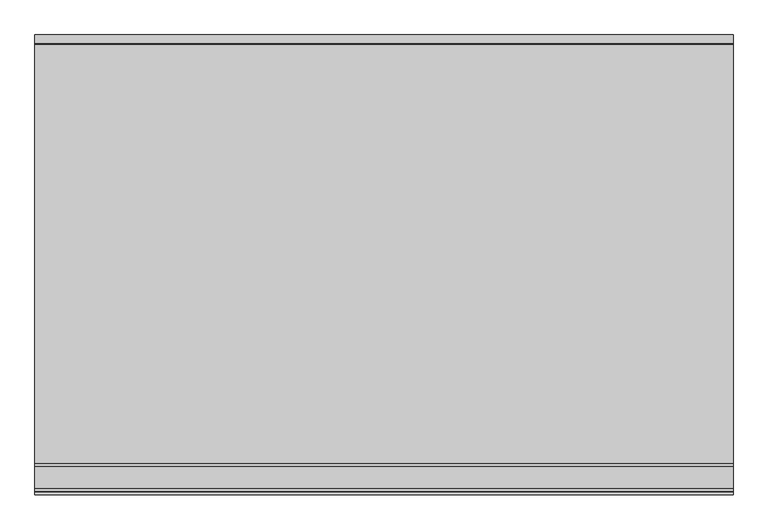
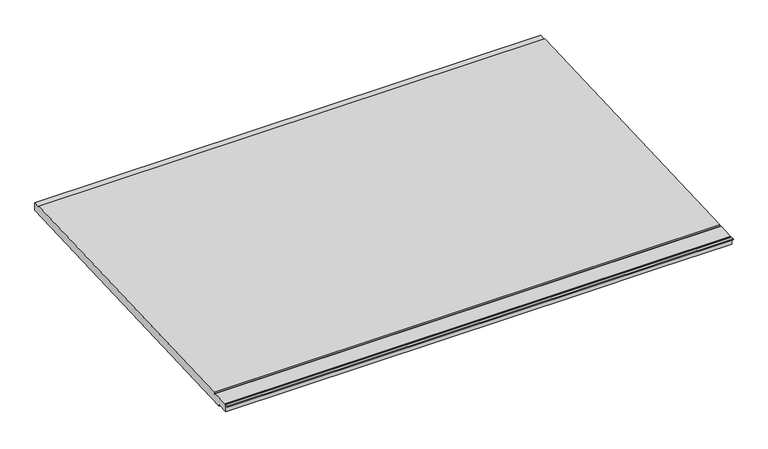
"""IFC4 building model written with IfcOpenShell, lengths in millimetres: proxy geometry, Generic Models 7:Generic Models 1:2:Generic Models 1:2 : Generic Models 7:Generic Models 1:337419:11 : Generic Models 7:Generic Models 1:2:Generic Models 1:2 : Generic Models 7:Generic Models 1:337419:306751."""

from ifc_helpers import new_model, si_unit, origin, place, context, project, spatial, faceted_brep, source, transform, mapped, element, save


def generic_models_fd5f59f4(model_context):
    return source(origin(), model_context, "Body", "Brep", [
        faceted_brep([(596182.8367239, -578988.1721757, 3950.4199851), (596182.8367239, -579061.0480378, 3947.3834909), (596182.8367239, -579059.461914, 3909.3165208), (596182.8367239, -578989.2957788, 3912.2401097), (596182.8367239, -578989.2957788, 3721.5748169), (596182.8367239, -578614.4804524, 3737.1921222), (596182.8367239, -578612.3656208, 3686.436162), (596182.8367239, -568205.6913841, 4120.0475886), (596182.8367239, -568205.6913841, 4374.267979), (596182.8367239, -568407.8188757, 4365.8460002), (596182.8367239, -568426.430308, 4390.492563), (596182.8367239, -578321.4396124, 3978.2005086), (596182.8367239, -578321.4396124, 3940.06745), (596182.8367239, -578397.8238233, 3936.8847746), (596182.8367239, -578397.8238233, 3975.0178331), (596182.8367239, -578911.9452054, 3953.5961089), (596182.8367239, -578910.3590816, 3915.5291388), (596182.8367239, -578986.5860519, 3912.353015), (579695.8219605, -579061.0480378, 3947.3834909), (579695.8219605, -578988.1721757, 3950.4199851), (579695.8219605, -578986.5860519, 3912.353015), (579695.8219605, -578910.3590816, 3915.5291388), (579695.8219605, -578911.9452054, 3953.5961089), (579695.8219605, -578397.8238233, 3975.0178331), (579695.8219605, -578397.8238233, 3936.8847746), (579695.8219605, -578321.4396124, 3940.06745), (579695.8219605, -578321.4396124, 3978.2005086), (579695.8219605, -568426.430308, 4390.492563), (579695.8219605, -568407.8188757, 4365.8460002), (579695.8219605, -568205.6913841, 4374.267979), (579695.8219605, -568205.6913841, 4120.0475886), (579695.8219605, -578612.3656208, 3686.436162), (579695.8219605, -578614.4804524, 3737.1921222), (579695.8219605, -578989.2957788, 3721.5748169), (579695.8219605, -578989.2957788, 3912.2401097), (579695.8219605, -579059.461914, 3909.3165208), (591306.0367239, -578989.2957788, 3721.5748169), (593738.0867239, -578989.2957788, 3721.5748169)], [[[0, 1, 2, 3, 4, 5, 6, 7, 8, 9, 10, 11, 12, 13, 14, 15, 16, 17]], [[18, 19, 20, 21, 22, 23, 24, 25, 26, 27, 28, 29, 30, 31, 32, 33, 34, 35]], [[1, 0, 19, 18]], [[9, 8, 29, 28]], [[10, 9, 28, 27]], [[8, 7, 30, 29]], [[7, 6, 31, 30]], [[2, 1, 18, 35]], [[3, 2, 35, 34]], [[4, 3, 34, 33, 36, 37]], [[5, 4, 37, 36, 33, 32]], [[6, 5, 32, 31]], [[15, 14, 23, 22]], [[16, 15, 22, 21]], [[17, 16, 21, 20]], [[0, 17, 20, 19]], [[11, 10, 27, 26]], [[12, 11, 26, 25]], [[13, 12, 25, 24]], [[14, 13, 24, 23]]]),
    ])


if __name__ == "__main__":
    model = new_model("IFC4")
    model_context = context("Model", 3, world=origin())
    ifc_project = project(units=[si_unit("LENGTHUNIT", "METRE", prefix="MILLI")], contexts=[model_context])
    site = spatial("IfcSite", under=ifc_project)
    building = spatial("IfcBuilding", under=site)
    placement = place(None, origin())
    generic_models_shape = generic_models_fd5f59f4(model_context)
    element("IfcBuildingElementProxy", 1, Name="Generic Models 7:Generic Models 1:2:Generic Models 1:2 : Generic Models 7:Generic Models 1:337419:11 : Generic Models 7:Generic Models 1:2:Generic Models 1:2 : Generic Models 7:Generic Models 1:337419:306751", ObjectType="Generic Models 7:Generic Models 1:2:Generic Models 1:2 : Generic Models 7:Generic Models 1:337419:11 : Generic Models 7:Generic Models 1:2:Generic Models 1:2 : Generic Models 7:Generic Models 1:337419:306751", at=placement, inside=building, context=model_context, shape_type="MappedRepresentation", body=[
        mapped(generic_models_shape, transform((0.0, 0.0, 0.0), x_axis=(1.0, 0.0, 0.0), y_axis=(0.0, 1.0, 0.0), z_axis=(0.0, 0.0, 1.0))),
    ])
    save(model, "model.ifc")

# Revit data of these elements
# Type "Generic Models 7:Generic Models 1:2:Generic Models 1:2 : Generic Models 7:Generic Models 1:337419:11 : Generic Models 7:Generic Models 1:2:Generic Models 1:2 : Generic Models 7:Generic Models 1:337419:306751"
#   NameOverride = "Generic Models 7:Generic Models 1:2:Generic Models 1:2 : Generic Models 7:Generic Models 1:337419:306751"
#   ObjectTypeOverride = "Generic Models 1:2 : Generic Models 7:Generic Models 1:337419"
#   Reference = "Generic Models 1"
#   Tag = "306751"
# Element 1 (IfcBuildingElementProxy, "Generic Models 7:Generic Models 1:2:Generic Models 1:2 : Generic Models 7:Generic Models 1:337419:11 : Generic Models 7:Generic Models 1:2:Generic Models 1:2 : Generic Models 7:Generic Models 1:337419:306751")
#   Materials on its faces: "FULL CAVITY CLASS A FIBERGLASS INSULATION WITH DURABLE VAPOR BARRIER (BLACK) LINER"
# Materials
#   "FULL CAVITY CLASS A FIBERGLASS INSULATION WITH DURABLE VAPOR BARRIER (BLACK) LINER": class "Unassigned", colour RGB 158 92 175, transparency 0, Cost = 0
